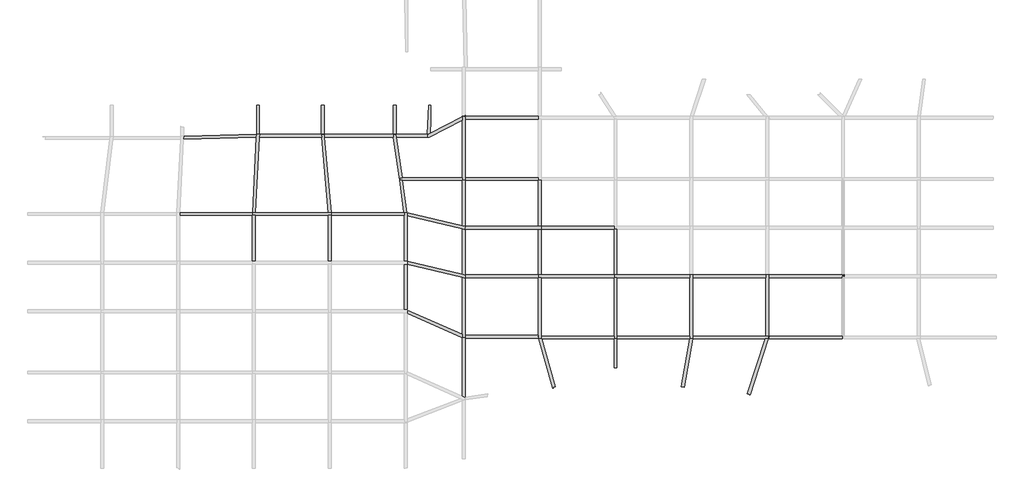
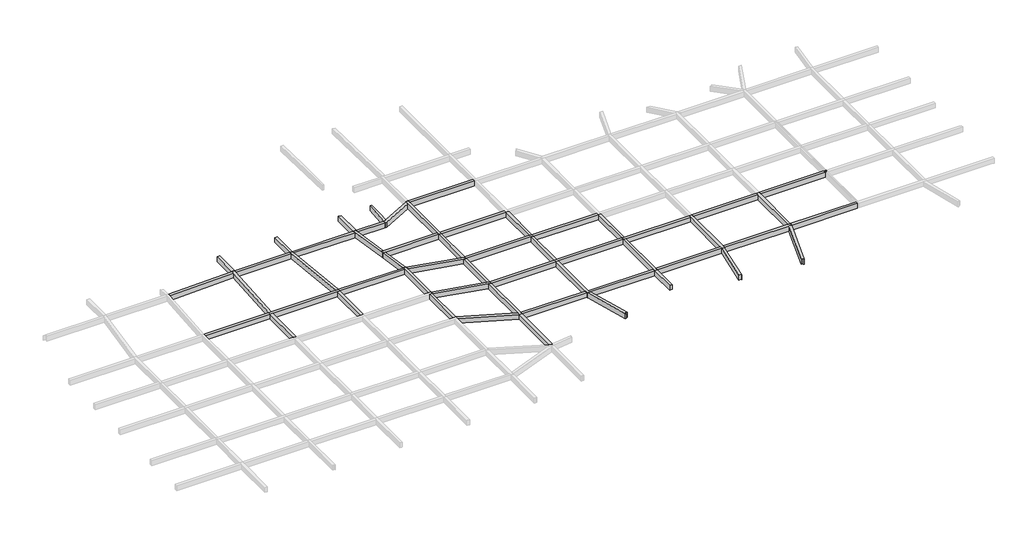
# One storey, part 8 of 15: 54 beams.
"""IFC4 building model written with IfcOpenShell, lengths in millimetres."""

from ifc_helpers import new_model, si_unit, frame, origin, place, context, project, spatial, polyline, outline, extrude, faceted_brep, element, save

model = new_model("IFC4")

# Units and contexts
model_context = context("Model", 3, world=origin())
ifc_project = project(units=[si_unit("LENGTHUNIT", "METRE", prefix="MILLI")], contexts=[model_context])

# Site, building, storey
site = spatial("IfcSite", under=ifc_project)
building = spatial("IfcBuilding", under=site)
storey = spatial("IfcBuildingStorey", under=building, Name="层高", Elevation=3300.0)

# Beams
placement = place(None, origin())
element("IfcBeam", 1, ObjectType="混凝土 - 矩形梁 : KL_beam", at=placement, inside=storey, context=model_context, shape_type="Brep", body=[
    faceted_brep([(131950.3009381, 116892.3894162, 3300.0), (131950.3009381, 116592.3894162, 3300.0), (132250.3009381, 116592.3894162, 3300.0), (139750.3009381, 116592.3894162, 3300.0), (140050.3009381, 116592.3894162, 3300.0), (140050.3009381, 116892.3894162, 3300.0), (140037.7506142, 116892.3894162, 3300.0), (139736.604663, 116892.3894162, 3300.0), (132258.3679569, 116892.3894162, 3300.0), (131957.9562531, 116892.3894162, 3300.0), (131950.3009381, 116592.3894162, 2700.0), (132250.3009381, 116592.3894162, 2700.0), (139750.3009381, 116592.3894162, 2700.0), (140050.3009381, 116592.3894162, 2700.0), (131950.3009381, 116892.3894162, 2700.0), (131957.9562531, 116892.3894162, 2700.0), (132258.3679569, 116892.3894162, 2700.0), (139736.604663, 116892.3894162, 2700.0), (140037.7506142, 116892.3894162, 2700.0), (140050.3009381, 116892.3894162, 2700.0)], [[[0, 1, 2, 3, 4, 5, 6, 7, 8, 9]], [[1, 10, 11, 12, 13, 4, 3, 2]], [[10, 14, 15, 16, 17, 18, 19, 13, 12, 11]], [[14, 0, 9, 8, 7, 6, 5, 19, 18, 17, 16, 15]], [[1, 0, 14, 10]], [[5, 4, 13, 19]]]),
])
element("IfcBeam", 2, ObjectType="混凝土 - 矩形梁 : KL_beam", at=placement, inside=storey, context=model_context, shape_type="SweptSolid", body=[
    extrude(outline(polyline([(131950.3009381, 116592.3894162), (132250.3009381, 116592.3894162), (132250.3009381, 111892.3894162), (131950.3009381, 111892.3894162), (131950.3009381, 116592.3894162)])), frame((0.0, 0.0, 2700.0), z_axis=(0.0, 0.0, 1.0), x_axis=(1.0, 0.0, 0.0)), (0.0, 0.0, 1.0), 600.0),
])
element("IfcBeam", 3, ObjectType="混凝土 - 矩形梁 : KL_beam", at=placement, inside=storey, context=model_context, shape_type="SweptSolid", body=[
    extrude(outline(polyline([(139750.3009381, 116592.3894162), (140050.3009381, 116592.3894162), (140050.3009381, 111892.3894162), (139750.3009381, 111892.3894162), (139750.3009381, 116592.3894162)])), frame((0.0, 0.0, 2700.0), z_axis=(0.0, 0.0, 1.0), x_axis=(1.0, 0.0, 0.0)), (0.0, 0.0, 1.0), 600.0),
])
element("IfcBeam", 4, ObjectType="混凝土 - 矩形梁 : KL_beam", at=placement, inside=storey, context=model_context, shape_type="Brep", body=[
    faceted_brep([(147850.2032763, 111592.3894162, 3300.0), (147550.2032763, 111592.3894162, 3300.0), (147550.2032763, 106892.3894162, 3300.0), (147850.2032763, 106892.3894162, 3300.0), (147850.2032763, 111553.3533934, 3300.0), (147550.2032763, 111592.3894162, 2700.0), (147550.2032763, 106892.3894162, 2700.0), (147850.2032763, 111592.3894162, 2700.0), (147850.2032763, 111553.3533934, 2700.0), (147850.2032763, 106892.3894162, 2700.0)], [[[0, 1, 2, 3, 4]], [[1, 5, 6, 2]], [[5, 7, 8, 9, 6]], [[7, 0, 4, 3, 9, 8]], [[1, 0, 7, 5]], [[3, 2, 6, 9]]]),
])
element("IfcBeam", 5, ObjectType="混凝土 - 矩形梁 : KL_beam", at=placement, inside=storey, context=model_context, shape_type="Brep", body=[
    faceted_brep([(147550.2032763, 111892.3894162, 2700.0), (147550.2032763, 111892.3894162, 3300.0), (147550.2032763, 116592.3894162, 3300.0), (147550.2032763, 116892.3894162, 3300.0), (147550.2032763, 116892.3894162, 2700.0), (147550.2032763, 116592.3894162, 2700.0), (147850.2032763, 111892.3894162, 3300.0), (147850.2032763, 111892.3894162, 2700.0), (147717.4740175, 116892.3894162, 3300.0), (147831.2059389, 116892.3894162, 3300.0), (147850.2032763, 116892.3894162, 3300.0), (147850.2032763, 116892.3894162, 2700.0), (147831.2059389, 116892.3894162, 2700.0), (147717.4740175, 116892.3894162, 2700.0), (147850.2032763, 116553.3533934, 3300.0), (147850.2032763, 116861.4143495, 3300.0), (147850.2032763, 116861.4143495, 2700.0), (147850.2032763, 116553.3533934, 2700.0)], [[[0, 1, 2, 3, 4, 5]], [[6, 1, 0, 7]], [[3, 8, 9, 10, 11, 12, 13, 4]], [[1, 6, 14, 15, 10, 9, 8, 3, 2]], [[7, 0, 5, 4, 13, 12, 11, 16, 17]], [[6, 7, 17, 16, 11, 10, 15, 14]]]),
])
element("IfcBeam", 6, ObjectType="混凝土 - 矩形梁 : KL_beam", at=placement, inside=storey, context=model_context, shape_type="Brep", body=[
    faceted_brep([(140050.3009381, 116892.3894162, 3300.0), (140050.3009381, 116592.3894162, 3300.0), (147550.2032763, 116592.3894162, 3300.0), (147550.2032763, 116892.3894162, 3300.0), (147528.451042, 116892.3894162, 3300.0), (140050.3009381, 116592.3894162, 2700.0), (147550.2032763, 116592.3894162, 2700.0), (140050.3009381, 116892.3894162, 2700.0), (147528.451042, 116892.3894162, 2700.0), (147550.2032763, 116892.3894162, 2700.0)], [[[0, 1, 2, 3, 4]], [[1, 5, 6, 2]], [[5, 7, 8, 9, 6]], [[7, 0, 4, 3, 9, 8]], [[1, 0, 7, 5]], [[3, 2, 6, 9]]]),
])
element("IfcBeam", 7, ObjectType="混凝土 - 矩形梁 : KL_beam", at=placement, inside=storey, context=model_context, shape_type="Brep", body=[
    faceted_brep([(147528.451042, 116892.3894162, 3300.0), (147550.2032763, 116892.3894162, 3300.0), (147717.4740175, 116892.3894162, 3300.0), (147522.2630229, 116937.9458643, 3300.0), (147717.4740175, 116892.3894162, 2700.0), (147522.2630229, 116937.9458643, 2700.0), (147550.2032763, 116892.3894162, 2700.0), (147528.451042, 116892.3894162, 2700.0)], [[[0, 1, 2, 3]], [[2, 4, 5, 3]], [[4, 6, 7, 5]], [[0, 7, 6, 4, 2, 1]], [[3, 5, 7, 0]]]),
    faceted_brep([(153782.1218117, 115169.0197936, 3300.0), (153683.0301969, 115192.1448334, 3300.0), (153550.3009381, 115223.1199001, 3300.0), (147850.2032763, 116553.3533934, 3300.0), (147850.2032763, 116553.3533934, 2700.0), (153550.3009381, 115223.1199001, 2700.0), (153683.0301969, 115192.1448334, 2700.0), (153782.1218117, 115169.0197936, 2700.0), (147850.2032763, 116861.4143495, 3300.0), (147850.2032763, 116861.4143495, 2700.0), (147850.2032763, 116592.3894162, 2700.0), (147850.2032763, 116592.3894162, 3300.0), (153787.5185091, 115192.1448334, 3300.0), (153850.3009381, 115461.1697666, 3300.0), (153550.3009381, 115531.1808562, 3300.0), (153850.3009381, 115461.1697666, 2700.0), (153550.3009381, 115531.1808562, 2700.0), (153787.5185091, 115192.1448334, 2700.0)], [[[0, 1, 2, 3, 4, 5, 6, 7]], [[8, 9, 10, 4, 3, 11]], [[3, 2, 1, 0, 12, 13, 14, 8, 11]], [[8, 14, 13, 15, 16, 9]], [[9, 16, 15, 17, 7, 6, 5, 4, 10]], [[0, 7, 17, 15, 13, 12]]]),
])
element("IfcBeam", 8, ObjectType="混凝土 - 矩形梁 : KL_beam", at=placement, inside=storey, context=model_context, shape_type="Brep", body=[
    faceted_brep([(147850.2032763, 111553.3533934, 3300.0), (147850.2032763, 111553.3533934, 2700.0), (153550.3009381, 110223.1199001, 2700.0), (153850.3009381, 110153.1088105, 2700.0), (153850.3009381, 110153.1088105, 3300.0), (153550.3009381, 110223.1199001, 3300.0), (147850.2032763, 111861.4143495, 3300.0), (147850.2032763, 111861.4143495, 2700.0), (147850.2032763, 111592.3894162, 2700.0), (147850.2032763, 111592.3894162, 3300.0), (153850.3009381, 110192.1448334, 3300.0), (153850.3009381, 110461.1697666, 3300.0), (153550.3009381, 110531.1808562, 3300.0), (153850.3009381, 110461.1697666, 2700.0), (153550.3009381, 110531.1808562, 2700.0), (153850.3009381, 110192.1448334, 2700.0)], [[[0, 1, 2, 3, 4, 5]], [[6, 7, 8, 1, 0, 9]], [[6, 9, 0, 5, 4, 10, 11, 12]], [[7, 6, 12, 11, 13, 14]], [[1, 8, 7, 14, 13, 15, 3, 2]], [[11, 10, 4, 3, 15, 13]]]),
])
element("IfcBeam", 9, ObjectType="混凝土 - 矩形梁 : KL_beam", at=placement, inside=storey, context=model_context, shape_type="Brep", body=[
    faceted_brep([(153550.3009381, 104021.0945528, 3300.0), (153850.3009381, 104021.0945528, 3300.0), (153850.3009381, 104269.2250309, 3300.0), (153850.3009381, 110153.1088105, 3300.0), (153550.3009381, 110223.1199001, 3300.0), (153550.3009381, 104348.5115934, 3300.0), (153850.3009381, 104021.0945528, 2700.0), (153850.3009381, 104269.2250309, 2700.0), (153850.3009381, 110153.1088105, 2700.0), (153550.3009381, 104021.0945528, 2700.0), (153550.3009381, 104348.5115934, 2700.0), (153550.3009381, 110223.1199001, 2700.0)], [[[0, 1, 2, 3, 4, 5]], [[1, 6, 7, 8, 3, 2]], [[6, 9, 10, 11, 8, 7]], [[9, 0, 5, 4, 11, 10]], [[4, 3, 8, 11]], [[0, 9, 6, 1]]]),
])
element("IfcBeam", 10, ObjectType="混凝土 - 矩形梁 : KL_beam", at=placement, inside=storey, context=model_context, shape_type="Brep", body=[
    faceted_brep([(147668.8470787, 106592.3894162, 3300.0), (147850.2032763, 106513.1028536, 3300.0), (153550.3009381, 104021.0945528, 3300.0), (153550.3009381, 104348.5115934, 3300.0), (147850.2032763, 106840.5198943, 3300.0), (147850.2032763, 106592.3894162, 3300.0), (147668.8470787, 106592.3894162, 2700.0), (147850.2032763, 106513.1028536, 2700.0), (153550.3009381, 104021.0945528, 2700.0), (147850.2032763, 106592.3894162, 2700.0), (147850.2032763, 106840.5198943, 2700.0), (153550.3009381, 104348.5115934, 2700.0)], [[[0, 1, 2, 3, 4, 5]], [[2, 1, 0, 6, 7, 8]], [[8, 7, 6, 9, 10, 11]], [[10, 4, 3, 11]], [[5, 9, 6, 0]], [[9, 5, 4, 10]], [[3, 2, 8, 11]]]),
])
element("IfcBeam", 11, ObjectType="混凝土 - 矩形梁 : KL_beam", at=placement, inside=storey, context=model_context, shape_type="Brep", body=[
    faceted_brep([(153850.3009381, 97839.1284443, 3300.0), (153850.3009381, 97914.6988398, 3300.0), (153850.3009381, 103969.2250309, 3300.0), (153850.3009381, 104021.0945528, 3300.0), (153550.3009381, 104021.0945528, 3300.0), (153550.3009381, 97974.1385386, 3300.0), (153550.3009381, 104021.0945528, 2700.0), (153550.3009381, 97974.1385386, 2700.0), (153850.3009381, 104021.0945528, 2700.0), (153850.3009381, 103969.2250309, 2700.0), (153850.3009381, 97914.6988398, 2700.0), (153850.3009381, 97839.1284443, 2700.0)], [[[0, 1, 2, 3, 4, 5]], [[4, 6, 7, 5]], [[8, 9, 10, 11, 7, 6]], [[3, 2, 1, 0, 11, 10, 9, 8]], [[4, 3, 8, 6]], [[0, 5, 7, 11]]]),
])
element("IfcBeam", 12, ObjectType="混凝土 - 矩形梁 : KL_beam", at=placement, inside=storey, context=model_context, shape_type="Brep", body=[
    faceted_brep([(177250.3009381, 110492.1448334, 3300.0), (176950.3009381, 110492.1448334, 3300.0), (176950.3009381, 110192.1448334, 3300.0), (176950.3009381, 104192.1448334, 3300.0), (176950.3009381, 103892.1448334, 3300.0), (177226.1658828, 103892.1448334, 3300.0), (177250.3009381, 103892.1448334, 3300.0), (177250.3009381, 104192.1448334, 3300.0), (177250.3009381, 110192.1448334, 3300.0), (177250.3009381, 110492.1448334, 2700.0), (177250.3009381, 103892.1448334, 2700.0), (177250.3009381, 104192.1448334, 2700.0), (177250.3009381, 110192.1448334, 2700.0), (176950.3009381, 110492.1448334, 2700.0), (177226.1658828, 103892.1448334, 2700.0), (176950.3009381, 103892.1448334, 2700.0), (176950.3009381, 104192.1448334, 2700.0), (176950.3009381, 110192.1448334, 2700.0)], [[[0, 1, 2, 3, 4, 5, 6, 7, 8]], [[9, 0, 8, 7, 6, 10, 11, 12]], [[13, 9, 12, 11, 10, 14, 15, 16, 17]], [[1, 13, 17, 16, 15, 4, 3, 2]], [[1, 0, 9, 13]], [[6, 5, 4, 15, 14, 10]]]),
])
element("IfcBeam", 13, ObjectType="混凝土 - 矩形梁 : KL_beam", at=placement, inside=storey, context=model_context, shape_type="Brep", body=[
    faceted_brep([(169150.3009381, 110492.1448334, 3300.0), (169150.3009381, 110192.1448334, 3300.0), (169450.3009381, 110192.1448334, 3300.0), (176950.3009381, 110192.1448334, 3300.0), (176950.3009381, 110492.1448334, 3300.0), (169450.3009381, 110492.1448334, 3300.0), (169150.3009381, 110492.1448334, 2700.0), (176950.3009381, 110492.1448334, 2700.0), (169450.3009381, 110492.1448334, 2700.0), (169150.3009381, 110192.1448334, 2700.0), (176950.3009381, 110192.1448334, 2700.0), (169450.3009381, 110192.1448334, 2700.0)], [[[0, 1, 2, 3, 4, 5]], [[6, 0, 5, 4, 7, 8]], [[9, 6, 8, 7, 10, 11]], [[1, 9, 11, 10, 3, 2]], [[4, 3, 10, 7]], [[1, 0, 6, 9]]]),
])
element("IfcBeam", 14, ObjectType="混凝土 - 矩形梁 : KL_beam", at=placement, inside=storey, context=model_context, shape_type="Brep", body=[
    faceted_brep([(169150.3009381, 103892.1448334, 3300.0), (169450.3009381, 103892.1448334, 3300.0), (169450.3009381, 104192.1448334, 3300.0), (169450.3009381, 110192.1448334, 3300.0), (169150.3009381, 110192.1448334, 3300.0), (169150.3009381, 104192.1448334, 3300.0), (169150.3009381, 103892.1448334, 2700.0), (169150.3009381, 110192.1448334, 2700.0), (169150.3009381, 104192.1448334, 2700.0), (169450.3009381, 103892.1448334, 2700.0), (169450.3009381, 110192.1448334, 2700.0), (169450.3009381, 104192.1448334, 2700.0)], [[[0, 1, 2, 3, 4, 5]], [[6, 0, 5, 4, 7, 8]], [[9, 6, 8, 7, 10, 11]], [[1, 9, 11, 10, 3, 2]], [[4, 3, 10, 7]], [[1, 0, 6, 9]]]),
])
element("IfcBeam", 15, ObjectType="混凝土 - 矩形梁 : KL_beam", at=placement, inside=storey, context=model_context, shape_type="Brep", body=[
    faceted_brep([(176950.3009381, 103892.1448334, 3300.0), (176950.3009381, 104192.1448334, 3300.0), (169450.3009381, 104192.1448334, 3300.0), (169450.3009381, 103892.1448334, 3300.0), (176921.5378992, 103892.1448334, 3300.0), (176950.3009381, 103892.1448334, 2700.0), (169450.3009381, 103892.1448334, 2700.0), (176921.5378992, 103892.1448334, 2700.0), (176950.3009381, 104192.1448334, 2700.0), (169450.3009381, 104192.1448334, 2700.0)], [[[0, 1, 2, 3, 4]], [[5, 0, 4, 3, 6, 7]], [[8, 5, 7, 6, 9]], [[1, 8, 9, 2]], [[1, 0, 5, 8]], [[3, 2, 9, 6]]]),
])
element("IfcBeam", 16, ObjectType="混凝土 - 矩形梁 : KL_beam", at=placement, inside=storey, context=model_context, shape_type="Brep", body=[
    faceted_brep([(177250.3009381, 104192.1448334, 3300.0), (177250.3009381, 103892.1448334, 3300.0), (184693.8920707, 103892.1448334, 3300.0), (185009.3078828, 103892.1448334, 3300.0), (185050.3009381, 103892.1448334, 3300.0), (185050.3009381, 104018.4043182, 3300.0), (185050.3009381, 104192.1448334, 3300.0), (184750.3009381, 104192.1448334, 3300.0), (177250.3009381, 103892.1448334, 2700.0), (184693.8920707, 103892.1448334, 2700.0), (185009.3078828, 103892.1448334, 2700.0), (185050.3009381, 103892.1448334, 2700.0), (177250.3009381, 104192.1448334, 2700.0), (184750.3009381, 104192.1448334, 2700.0), (185050.3009381, 104192.1448334, 2700.0), (185050.3009381, 104018.4043182, 2700.0)], [[[0, 1, 2, 3, 4, 5, 6, 7]], [[1, 8, 9, 10, 11, 4, 3, 2]], [[8, 12, 13, 14, 15, 11, 10, 9]], [[12, 0, 7, 6, 14, 13]], [[1, 0, 12, 8]], [[6, 5, 4, 11, 15, 14]]]),
])
element("IfcBeam", 17, ObjectType="混凝土 - 矩形梁 : KL_beam", at=placement, inside=storey, context=model_context, shape_type="Brep", body=[
    faceted_brep([(185050.3009381, 110492.1448334, 3300.0), (184750.3009381, 110492.1448334, 3300.0), (184750.3009381, 110192.1448334, 3300.0), (184750.3009381, 104192.1448334, 3300.0), (185050.3009381, 104192.1448334, 3300.0), (185050.3009381, 110192.1448334, 3300.0), (184750.3009381, 110492.1448334, 2700.0), (184750.3009381, 110192.1448334, 2700.0), (184750.3009381, 104192.1448334, 2700.0), (185050.3009381, 110492.1448334, 2700.0), (185050.3009381, 110192.1448334, 2700.0), (185050.3009381, 104192.1448334, 2700.0)], [[[0, 1, 2, 3, 4, 5]], [[1, 6, 7, 8, 3, 2]], [[6, 9, 10, 11, 8, 7]], [[9, 0, 5, 4, 11, 10]], [[4, 3, 8, 11]], [[1, 0, 9, 6]]]),
])
element("IfcBeam", 18, ObjectType="混凝土 - 矩形梁 : KL_beam", at=placement, inside=storey, context=model_context, shape_type="SweptSolid", body=[
    extrude(outline(polyline([(177250.3009381, 110192.1448334), (177250.3009381, 110492.1448334), (184750.3009381, 110492.1448334), (184750.3009381, 110192.1448334), (177250.3009381, 110192.1448334)])), frame((0.0, 0.0, 2700.0), z_axis=(0.0, 0.0, 1.0), x_axis=(1.0, 0.0, 0.0)), (0.0, 0.0, 1.0), 600.0),
])
element("IfcBeam", 19, ObjectType="混凝土 - 矩形梁 : KL_beam", at=placement, inside=storey, context=model_context, shape_type="SweptSolid", body=[
    extrude(outline(polyline([(169450.3009381, 110492.1448334), (169150.3009381, 110492.1448334), (169150.3009381, 115192.1448334), (169450.3009381, 115192.1448334), (169450.3009381, 110492.1448334)])), frame((0.0, 0.0, 2700.0), z_axis=(0.0, 0.0, 1.0), x_axis=(1.0, 0.0, 0.0)), (0.0, 0.0, 1.0), 600.0),
])
element("IfcBeam", 20, ObjectType="混凝土 - 矩形梁 : KL_beam", at=placement, inside=storey, context=model_context, shape_type="Brep", body=[
    faceted_brep([(161350.3009383, 110492.1448334, 3300.0), (161350.3009383, 110192.1448334, 3300.0), (161650.3009383, 110192.1448334, 3300.0), (169150.3009381, 110192.1448334, 3300.0), (169150.3009381, 110492.1448334, 3300.0), (161650.3009383, 110492.1448334, 3300.0), (161350.3009383, 110192.1448334, 2700.0), (161650.3009383, 110192.1448334, 2700.0), (169150.3009381, 110192.1448334, 2700.0), (161350.3009383, 110492.1448334, 2700.0), (161650.3009383, 110492.1448334, 2700.0), (169150.3009381, 110492.1448334, 2700.0)], [[[0, 1, 2, 3, 4, 5]], [[1, 6, 7, 8, 3, 2]], [[6, 9, 10, 11, 8, 7]], [[9, 0, 5, 4, 11, 10]], [[4, 3, 8, 11]], [[1, 0, 9, 6]]]),
])
element("IfcBeam", 21, ObjectType="混凝土 - 矩形梁 : KL_beam", at=placement, inside=storey, context=model_context, shape_type="Brep", body=[
    faceted_brep([(161350.3009383, 103892.1448334, 3300.0), (161387.2678308, 103892.1448334, 3300.0), (161650.3009383, 103892.1448334, 3300.0), (161650.3009383, 104192.1448334, 3300.0), (161650.3009383, 110192.1448334, 3300.0), (161350.3009383, 110192.1448334, 3300.0), (161350.3009383, 104269.2250309, 3300.0), (161350.3009383, 104208.7009636, 3300.0), (161350.3009383, 104021.0637081, 3300.0), (161350.3009383, 103969.2250309, 3300.0), (161650.3009383, 103892.1448334, 2700.0), (161650.3009383, 104192.1448334, 2700.0), (161650.3009383, 110192.1448334, 2700.0), (161387.2678308, 103892.1448334, 2700.0), (161350.3009383, 103892.1448334, 2700.0), (161350.3009383, 103969.2250309, 2700.0), (161350.3009383, 104021.0637081, 2700.0), (161350.3009383, 104208.7009636, 2700.0), (161350.3009383, 104269.2250309, 2700.0), (161350.3009383, 110192.1448334, 2700.0)], [[[0, 1, 2, 3, 4, 5, 6, 7, 8, 9]], [[2, 10, 11, 12, 4, 3]], [[10, 13, 14, 15, 16, 17, 18, 19, 12, 11]], [[14, 0, 9, 8, 7, 6, 5, 19, 18, 17, 16, 15]], [[5, 4, 12, 19]], [[2, 1, 0, 14, 13, 10]]]),
])
element("IfcBeam", 22, ObjectType="混凝土 - 矩形梁 : KL_beam", at=placement, inside=storey, context=model_context, shape_type="Brep", body=[
    faceted_brep([(169150.3009381, 103892.1448334, 3300.0), (169150.3009381, 104192.1448334, 3300.0), (161650.3009383, 104192.1448334, 3300.0), (161650.3009383, 103892.1448334, 3300.0), (161699.3576615, 103892.1448334, 3300.0), (169150.3009381, 104192.1448334, 2700.0), (161650.3009383, 104192.1448334, 2700.0), (169150.3009381, 103892.1448334, 2700.0), (161699.3576615, 103892.1448334, 2700.0), (161650.3009383, 103892.1448334, 2700.0)], [[[0, 1, 2, 3, 4]], [[1, 5, 6, 2]], [[5, 7, 8, 9, 6]], [[7, 0, 4, 3, 9, 8]], [[1, 0, 7, 5]], [[3, 2, 6, 9]]]),
])
element("IfcBeam", 23, ObjectType="混凝土 - 矩形梁 : KL_beam", at=placement, inside=storey, context=model_context, shape_type="Brep", body=[
    faceted_brep([(161699.3576615, 103892.1448334, 3300.0), (161650.3009383, 103892.1448334, 3300.0), (161387.2678308, 103892.1448334, 3300.0), (162838.6902887, 98830.4331897, 3300.0), (162917.5304809, 98830.4331897, 3300.0), (162917.5304809, 98950.4331897, 3300.0), (163116.3706731, 98950.4331897, 3300.0), (161387.2678308, 103892.1448334, 2700.0), (162838.6902887, 98830.4331897, 2700.0), (161650.3009383, 103892.1448334, 2700.0), (161699.3576615, 103892.1448334, 2700.0), (163116.3706731, 98950.4331897, 2700.0), (162917.5304809, 98950.4331897, 2700.0), (162917.5304809, 98830.4331897, 2700.0)], [[[0, 1, 2, 3, 4, 5, 6]], [[2, 7, 8, 3]], [[7, 9, 10, 11, 12, 13, 8]], [[10, 0, 6, 11]], [[7, 2, 1, 0, 10, 9]], [[3, 8, 13, 4]], [[5, 12, 11, 6]], [[12, 5, 4, 13]]]),
    faceted_brep([(161300.5846401, 104194.4450445, 2700.0), (161300.5846401, 104194.4450445, 3300.0), (161350.3009383, 104208.7009636, 3300.0), (161350.3009383, 104208.7009636, 2700.0), (161350.3009383, 104021.0637081, 3300.0), (161350.3009383, 104021.0637081, 2700.0), (161350.3009383, 104192.1448334, 2700.0), (161350.3009383, 104192.1448334, 3300.0)], [[[0, 1, 2, 3]], [[4, 5, 6, 3, 2, 7]], [[2, 1, 4, 7]], [[1, 0, 5, 4]], [[0, 3, 6, 5]]]),
])
element("IfcBeam", 24, ObjectType="混凝土 - 矩形梁 : KL_beam", at=placement, inside=storey, context=model_context, shape_type="SweptSolid", body=[
    extrude(outline(polyline([(169150.3009381, 103892.1448334), (169450.3009381, 103892.1448334), (169450.3009381, 100902.3018651), (169150.3009381, 100902.3018651), (169150.3009381, 103892.1448334)])), frame((0.0, 0.0, 2700.0), z_axis=(0.0, 0.0, 1.0), x_axis=(1.0, 0.0, 0.0)), (0.0, 0.0, 1.0), 600.0),
])
element("IfcBeam", 25, ObjectType="混凝土 - 矩形梁 : KL_beam", at=placement, inside=storey, context=model_context, shape_type="Brep", body=[
    faceted_brep([(177226.1658828, 103892.1448334, 3300.0), (176950.3009381, 103892.1448334, 3300.0), (176921.5378992, 103892.1448334, 3300.0), (176050.1808056, 98950.4331897, 3300.0), (176349.86269, 98950.4331897, 3300.0), (176349.86269, 98922.3824677, 3300.0), (176921.5378992, 103892.1448334, 2700.0), (176050.1808056, 98950.4331897, 2700.0), (176950.3009381, 103892.1448334, 2700.0), (177226.1658828, 103892.1448334, 2700.0), (176349.86269, 98922.3824677, 2700.0), (176349.86269, 98950.4331897, 2700.0)], [[[0, 1, 2, 3, 4, 5]], [[2, 6, 7, 3]], [[6, 8, 9, 10, 11, 7]], [[9, 0, 5, 10]], [[0, 9, 8, 6, 2, 1]], [[3, 7, 11, 4]], [[4, 11, 10, 5]]]),
])
element("IfcBeam", 26, ObjectType="混凝土 - 矩形梁 : KL_beam", at=placement, inside=storey, context=model_context, shape_type="Brep", body=[
    faceted_brep([(185050.3009381, 104192.1448334, 3300.0), (185050.3009381, 104018.4043182, 3300.0), (185106.7098056, 104192.1448334, 3300.0), (185050.3009381, 104018.4043182, 2700.0), (185106.7098056, 104192.1448334, 2700.0), (185050.3009381, 104192.1448334, 2700.0)], [[[0, 1, 2]], [[1, 3, 4, 2]], [[3, 5, 4]], [[5, 0, 2, 4]], [[1, 0, 5, 3]]]),
    faceted_brep([(184693.8920707, 103892.1448334, 3300.0), (184693.8920707, 103892.1448334, 2700.0), (182862.1801986, 98250.4331897, 2700.0), (182862.1801986, 98250.4331897, 3300.0), (185009.3078828, 103892.1448334, 3300.0), (185009.3078828, 103892.1448334, 2700.0), (184750.3009381, 103892.1448334, 2700.0), (184750.3009381, 103892.1448334, 3300.0), (183060.4077201, 98250.4331897, 3300.0), (183060.4077201, 98130.4331897, 3300.0), (183138.6352416, 98130.4331897, 3300.0), (183138.6352416, 98130.4331897, 2700.0), (183060.4077201, 98130.4331897, 2700.0), (183060.4077201, 98250.4331897, 2700.0)], [[[0, 1, 2, 3]], [[4, 5, 6, 1, 0, 7]], [[7, 0, 3, 8, 9, 10, 4]], [[5, 4, 10, 11]], [[6, 5, 11, 12, 13, 2, 1]], [[11, 10, 9, 12]], [[8, 13, 12, 9]], [[13, 8, 3, 2]]]),
])
element("IfcBeam", 27, ObjectType="混凝土 - 矩形梁 : KL_beam", at=placement, inside=storey, context=model_context, shape_type="Brep", body=[
    faceted_brep([(185050.3009381, 104018.4043182, 3300.0), (185050.3009381, 103892.1448334, 3300.0), (192640.3009401, 103892.1448334, 3300.0), (192640.3009401, 104192.1448334, 3300.0), (192550.3215993, 104192.1448334, 3300.0), (185106.7098056, 104192.1448334, 3300.0), (185050.3009381, 103892.1448334, 2700.0), (192640.3009401, 103892.1448334, 2700.0), (185050.3009381, 104018.4043182, 2700.0), (185106.7098056, 104192.1448334, 2700.0), (192550.3215993, 104192.1448334, 2700.0), (192640.3009401, 104192.1448334, 2700.0)], [[[0, 1, 2, 3, 4, 5]], [[1, 6, 7, 2]], [[6, 8, 9, 10, 11, 7]], [[9, 5, 4, 3, 11, 10]], [[6, 1, 0, 8]], [[0, 5, 9, 8]], [[3, 2, 7, 11]]]),
])
element("IfcBeam", 28, ObjectType="混凝土 - 矩形梁 : KL_beam", at=placement, inside=storey, context=model_context, shape_type="Brep", body=[
    faceted_brep([(192850.3009401, 110342.1448334, 3300.0), (192850.3009401, 110492.1448334, 3300.0), (192760.3009401, 110492.1448334, 3300.0), (192760.3009401, 110342.1448334, 3300.0), (192850.3009401, 110492.1448334, 2700.0), (192850.3009401, 110342.1448334, 2700.0), (192760.3009401, 110342.1448334, 2700.0), (192760.3009401, 110492.1448334, 2700.0)], [[[0, 1, 2, 3]], [[4, 5, 6, 7]], [[1, 4, 7, 2]], [[4, 1, 0, 5]], [[3, 2, 7, 6]], [[5, 0, 3, 6]]]),
    faceted_brep([(185050.3009381, 110192.1448334, 3300.0), (185050.3009381, 110192.1448334, 2700.0), (192550.3215993, 110192.1448334, 2700.0), (192550.3215993, 110192.1448334, 3300.0), (185050.3009381, 110492.1448334, 3300.0), (185050.3009381, 110492.1448334, 2700.0), (192550.3215993, 110342.1448334, 3300.0), (192550.3215993, 110342.1448334, 2700.0), (192640.3009401, 110342.1448334, 2700.0), (192640.3009401, 110342.1448334, 3300.0), (192640.3009401, 110492.1448334, 3300.0), (192640.3009401, 110492.1448334, 2700.0), (192550.3009401, 110492.1448334, 3300.0), (192550.3009401, 110492.1448334, 2700.0)], [[[0, 1, 2, 3]], [[0, 4, 5, 1]], [[6, 3, 2, 7]], [[6, 7, 8, 9]], [[10, 9, 8, 11]], [[4, 0, 3, 6, 9, 10, 12]], [[1, 5, 13, 11, 8, 7, 2]], [[5, 4, 12, 10, 11, 13]]]),
])
element("IfcBeam", 29, ObjectType="混凝土 - 矩形梁 : KL_beam", at=placement, inside=storey, context=model_context, shape_type="Brep", body=[
    faceted_brep([(153850.3009381, 126792.1448334, 3300.0), (153664.2891243, 126792.1448334, 3300.0), (153550.3009381, 126792.1448334, 3300.0), (153550.3009381, 126734.0649516, 3300.0), (153550.3009381, 126397.3670803, 3300.0), (153550.3009381, 120492.1448334, 3300.0), (153550.3009381, 120192.1448334, 3300.0), (153850.3009381, 120192.1448334, 3300.0), (153850.3009381, 120492.1448334, 3300.0), (153850.3009381, 126492.1448334, 3300.0), (153550.3009381, 126792.1448334, 2700.0), (153550.3009381, 126734.0649516, 2700.0), (153550.3009381, 126397.3670803, 2700.0), (153550.3009381, 120492.1448334, 2700.0), (153550.3009381, 120192.1448334, 2700.0), (153664.2891243, 126792.1448334, 2700.0), (153850.3009381, 126792.1448334, 2700.0), (153850.3009381, 126492.1448334, 2700.0), (153850.3009381, 120492.1448334, 2700.0), (153850.3009381, 120192.1448334, 2700.0)], [[[0, 1, 2, 3, 4, 5, 6, 7, 8, 9]], [[2, 10, 11, 12, 13, 14, 6, 5, 4, 3]], [[10, 15, 16, 17, 18, 19, 14, 13, 12, 11]], [[16, 0, 9, 8, 7, 19, 18, 17]], [[2, 1, 0, 16, 15, 10]], [[7, 6, 14, 19]]]),
])
element("IfcBeam", 30, ObjectType="混凝土 - 矩形梁 : KL_beam", at=placement, inside=storey, context=model_context, shape_type="SweptSolid", body=[
    extrude(outline(polyline([(161350.3009383, 126792.1448334), (161350.3009383, 126492.1448334), (153850.3009381, 126492.1448334), (153850.3009381, 126792.1448334), (161350.3009383, 126792.1448334)])), frame((0.0, 0.0, 2700.0), z_axis=(0.0, 0.0, 1.0), x_axis=(1.0, 0.0, 0.0)), (0.0, 0.0, 1.0), 600.0),
])
element("IfcBeam", 31, ObjectType="混凝土 - 矩形梁 : KL_beam", at=placement, inside=storey, context=model_context, shape_type="SweptSolid", body=[
    extrude(outline(polyline([(161350.3009383, 120492.1448334), (161350.3009383, 120192.1448334), (153850.3009381, 120192.1448334), (153850.3009381, 120492.1448334), (161350.3009383, 120492.1448334)])), frame((0.0, 0.0, 2700.0), z_axis=(0.0, 0.0, 1.0), x_axis=(1.0, 0.0, 0.0)), (0.0, 0.0, 1.0), 600.0),
])
element("IfcBeam", 32, ObjectType="混凝土 - 矩形梁 : KL_beam", at=placement, inside=storey, context=model_context, shape_type="Brep", body=[
    faceted_brep([(147080.2389772, 120492.1448334, 3300.0), (147080.2389772, 120196.4827327, 3300.0), (147080.2389772, 120192.1448334, 3300.0), (147382.9938741, 120192.1448334, 3300.0), (153550.3009381, 120192.1448334, 3300.0), (153550.3009381, 120492.1448334, 3300.0), (147341.6346506, 120492.1448334, 3300.0), (147080.2389772, 120192.1448334, 2700.0), (147382.9938741, 120192.1448334, 2700.0), (153550.3009381, 120192.1448334, 2700.0), (147080.2389772, 120196.4827327, 2700.0), (147080.2389772, 120492.1448334, 2700.0), (147341.6346506, 120492.1448334, 2700.0), (153550.3009381, 120492.1448334, 2700.0)], [[[0, 1, 2, 3, 4, 5, 6]], [[2, 7, 8, 9, 4, 3]], [[7, 10, 11, 12, 13, 9, 8]], [[11, 0, 6, 5, 13, 12]], [[5, 4, 9, 13]], [[0, 11, 10, 7, 2, 1]]]),
])
element("IfcBeam", 33, ObjectType="混凝土 - 矩形梁 : KL_beam", at=placement, inside=storey, context=model_context, shape_type="SweptSolid", body=[
    extrude(outline(polyline([(147831.2059389, 116892.3894162), (147717.4740175, 116892.3894162), (147522.2630229, 116937.9458643), (147080.2389772, 120192.1448334), (147382.9938741, 120192.1448334), (147831.2059389, 116892.3894162)])), frame((0.0, 0.0, 2700.0), z_axis=(0.0, 0.0, 1.0), x_axis=(1.0, 0.0, 0.0)), (0.0, 0.0, 1.0), 600.0),
])
element("IfcBeam", 34, ObjectType="混凝土 - 矩形梁 : KL_beam", at=placement, inside=storey, context=model_context, shape_type="Brep", body=[
    faceted_brep([(153550.3009381, 115531.1808562, 3300.0), (153850.3009381, 115461.1697666, 3300.0), (153850.3009381, 115492.1448334, 3300.0), (153850.3009381, 120192.1448334, 3300.0), (153550.3009381, 120192.1448334, 3300.0), (153850.3009381, 115461.1697666, 2700.0), (153850.3009381, 115492.1448334, 2700.0), (153850.3009381, 120192.1448334, 2700.0), (153550.3009381, 115531.1808562, 2700.0), (153550.3009381, 120192.1448334, 2700.0)], [[[0, 1, 2, 3, 4]], [[1, 5, 6, 7, 3, 2]], [[5, 8, 9, 7, 6]], [[8, 0, 4, 9]], [[1, 0, 8, 5]], [[4, 3, 7, 9]]]),
])
element("IfcBeam", 35, ObjectType="混凝土 - 矩形梁 : KL_beam", at=placement, inside=storey, context=model_context, shape_type="Brep", body=[
    faceted_brep([(153850.3009381, 115461.1697666, 3300.0), (153787.5185091, 115192.1448334, 3300.0), (153850.3009381, 115192.1448334, 3300.0), (161350.3009383, 115192.1448334, 3300.0), (161650.3009383, 115192.1448334, 3300.0), (161650.3009383, 115492.1448334, 3300.0), (161350.3009383, 115492.1448334, 3300.0), (153850.3009381, 115492.1448334, 3300.0), (161650.3009383, 115492.1448334, 2700.0), (161350.3009383, 115492.1448334, 2700.0), (153850.3009381, 115492.1448334, 2700.0), (153787.5185091, 115192.1448334, 2700.0), (153850.3009381, 115461.1697666, 2700.0), (161650.3009383, 115192.1448334, 2700.0), (161350.3009383, 115192.1448334, 2700.0), (153850.3009381, 115192.1448334, 2700.0)], [[[0, 1, 2, 3, 4, 5, 6, 7]], [[5, 8, 9, 10, 7, 6]], [[11, 12, 10, 9, 8, 13, 14, 15]], [[1, 11, 15, 14, 13, 4, 3, 2]], [[1, 0, 12, 11]], [[0, 7, 10, 12]], [[5, 4, 13, 8]]]),
    faceted_brep([(153550.3009381, 115223.1199001, 3300.0), (153683.0301969, 115192.1448334, 3300.0), (153683.0301969, 115192.1448334, 2700.0), (153550.3009381, 115223.1199001, 2700.0), (153550.3009381, 115192.1448334, 2700.0), (153550.3009381, 115192.1448334, 3300.0)], [[[0, 1, 2, 3]], [[4, 5, 0, 3]], [[1, 0, 5]], [[3, 2, 4]], [[2, 1, 5, 4]]]),
])
element("IfcBeam", 36, ObjectType="混凝土 - 矩形梁 : KL_beam", at=placement, inside=storey, context=model_context, shape_type="Brep", body=[
    faceted_brep([(153787.5185091, 115192.1448334, 3300.0), (153782.1218117, 115169.0197936, 3300.0), (153683.0301969, 115192.1448334, 3300.0), (153550.3009381, 115192.1448334, 3300.0), (153550.3009381, 110531.1808562, 3300.0), (153850.3009381, 110461.1697666, 3300.0), (153850.3009381, 110492.1448334, 3300.0), (153850.3009381, 115192.1448334, 3300.0), (153550.3009381, 115192.1448334, 2700.0), (153550.3009381, 110531.1808562, 2700.0), (153683.0301969, 115192.1448334, 2700.0), (153782.1218117, 115169.0197936, 2700.0), (153787.5185091, 115192.1448334, 2700.0), (153850.3009381, 115192.1448334, 2700.0), (153850.3009381, 110492.1448334, 2700.0), (153850.3009381, 110461.1697666, 2700.0)], [[[0, 1, 2, 3, 4, 5, 6, 7]], [[3, 8, 9, 4]], [[10, 11, 12, 13, 14, 15, 9, 8]], [[13, 7, 6, 5, 15, 14]], [[1, 11, 10, 2]], [[11, 1, 0, 12]], [[3, 2, 10, 8]], [[0, 7, 13, 12]], [[5, 4, 9, 15]]]),
])
element("IfcBeam", 37, ObjectType="混凝土 - 矩形梁 : KL_beam", at=placement, inside=storey, context=model_context, shape_type="Brep", body=[
    faceted_brep([(153850.3009381, 110492.1448334, 2700.0), (153850.3009381, 110492.1448334, 3300.0), (161350.3009383, 110492.1448334, 3300.0), (161350.3009383, 110492.1448334, 2700.0), (153850.3009381, 110192.1448334, 2700.0), (153850.3009381, 110192.1448334, 3300.0), (153850.3009381, 110461.1697666, 3300.0), (153850.3009381, 110461.1697666, 2700.0), (161350.3009383, 110192.1448334, 3300.0), (161350.3009383, 110192.1448334, 2700.0)], [[[0, 1, 2, 3]], [[4, 5, 6, 1, 0, 7]], [[1, 6, 5, 8, 2]], [[5, 4, 9, 8]], [[4, 7, 0, 3, 9]], [[3, 2, 8, 9]]]),
])
element("IfcBeam", 38, ObjectType="混凝土 - 矩形梁 : KL_beam", at=placement, inside=storey, context=model_context, shape_type="SweptSolid", body=[
    extrude(outline(polyline([(161650.3009383, 110492.1448334), (161350.3009383, 110492.1448334), (161350.3009383, 115192.1448334), (161650.3009383, 115192.1448334), (161650.3009383, 110492.1448334)])), frame((0.0, 0.0, 2700.0), z_axis=(0.0, 0.0, 1.0), x_axis=(1.0, 0.0, 0.0)), (0.0, 0.0, 1.0), 600.0),
])
element("IfcBeam", 39, ObjectType="混凝土 - 矩形梁 : KL_beam", at=placement, inside=storey, context=model_context, shape_type="Brep", body=[
    faceted_brep([(153850.3009381, 104269.2250309, 2700.0), (153850.3009381, 104269.2250309, 3300.0), (161350.3009383, 104269.2250309, 3300.0), (161350.3009383, 104269.2250309, 2700.0), (153850.3009381, 104021.0945528, 2700.0), (153850.3009381, 103969.2250309, 2700.0), (153850.3009381, 103969.2250309, 3300.0), (153850.3009381, 104021.0945528, 3300.0), (161350.3009383, 104208.7009636, 3300.0), (161350.3009383, 104208.7009636, 2700.0), (161350.3009383, 103969.2250309, 3300.0), (161350.3009383, 104021.0637081, 3300.0), (161300.5846401, 104194.4450445, 3300.0), (161350.3009383, 103969.2250309, 2700.0), (161300.5846401, 104194.4450445, 2700.0), (161350.3009383, 104021.0637081, 2700.0)], [[[0, 1, 2, 3]], [[1, 0, 4, 5, 6, 7]], [[3, 2, 8, 9]], [[1, 7, 6, 10, 11, 12, 8, 2]], [[6, 5, 13, 10]], [[5, 4, 0, 3, 9, 14, 15, 13]], [[14, 12, 11, 15]], [[12, 14, 9, 8]], [[10, 13, 15, 11]]]),
])
element("IfcBeam", 40, ObjectType="混凝土 - 矩形梁 : KL_beam", at=placement, inside=storey, context=model_context, shape_type="SweptSolid", body=[
    extrude(outline(polyline([(124450.3009381, 116592.3894162), (124450.3009381, 116738.461528), (124458.3679569, 116892.3894162), (131950.3009381, 116892.3894162), (131950.3009381, 116592.3894162), (124450.3009381, 116592.3894162)])), frame((0.0, 0.0, 2700.0), z_axis=(0.0, 0.0, 1.0), x_axis=(1.0, 0.0, 0.0)), (0.0, 0.0, 1.0), 600.0),
])
element("IfcBeam", 41, ObjectType="混凝土 - 矩形梁 : KL_beam", at=placement, inside=storey, context=model_context, shape_type="Brep", body=[
    faceted_brep([(131957.9562531, 116892.3894162, 3300.0), (132250.3009381, 116892.3894162, 3300.0), (132258.3679569, 116892.3894162, 3300.0), (132664.8406872, 124648.3511427, 3300.0), (132680.563021, 124948.3511427, 3300.0), (132672.4960022, 124948.3511427, 3300.0), (132520.2611111, 124948.3511427, 3300.0), (132380.1513172, 124948.3511427, 3300.0), (132379.9321201, 124944.1686142, 3300.0), (132364.1781965, 124643.5658433, 3300.0), (132258.3679569, 116892.3894162, 2700.0), (132664.8406872, 124648.3511427, 2700.0), (132680.563021, 124948.3511427, 2700.0), (132250.3009381, 116892.3894162, 2700.0), (131957.9562531, 116892.3894162, 2700.0), (132364.1781965, 124643.5658433, 2700.0), (132379.9321201, 124944.1686142, 2700.0), (132380.1513172, 124948.3511427, 2700.0), (132520.2611111, 124948.3511427, 2700.0), (132672.4960022, 124948.3511427, 2700.0)], [[[0, 1, 2, 3, 4, 5, 6, 7, 8, 9]], [[2, 10, 11, 12, 4, 3]], [[10, 13, 14, 15, 16, 17, 18, 19, 12, 11]], [[14, 0, 9, 8, 7, 17, 16, 15]], [[10, 2, 1, 0, 14, 13]], [[7, 6, 5, 4, 12, 19, 18, 17]]]),
])
element("IfcBeam", 42, ObjectType="混凝土 - 矩形梁 : KL_beam", at=placement, inside=storey, context=model_context, shape_type="Brep", body=[
    faceted_brep([(139034.0868799, 124922.2044199, 3300.0), (139058.0459371, 124648.3511427, 3300.0), (139736.604663, 116892.3894162, 3300.0), (139750.3009381, 116892.3894162, 3300.0), (140037.7506142, 116892.3894162, 3300.0), (139359.1918884, 124648.3511427, 3300.0), (139332.9452894, 124948.3511427, 3300.0), (140037.7506142, 116892.3894162, 2700.0), (139359.1918884, 124648.3511427, 2700.0), (139332.9452894, 124948.3511427, 2700.0), (139750.3009381, 116892.3894162, 2700.0), (139736.604663, 116892.3894162, 2700.0), (139058.0459371, 124648.3511427, 2700.0), (139034.0868799, 124922.2044199, 2700.0)], [[[0, 1, 2, 3, 4, 5, 6]], [[6, 5, 4, 7, 8, 9]], [[9, 8, 7, 10, 11, 12, 13]], [[2, 1, 0, 13, 12, 11]], [[7, 4, 3, 2, 11, 10]], [[0, 6, 9, 13]]]),
])
element("IfcBeam", 43, ObjectType="混凝土 - 矩形梁 : KL_beam", at=placement, inside=storey, context=model_context, shape_type="Brep", body=[
    faceted_brep([(146418.2752756, 124906.5992124, 3300.0), (146454.5696749, 124648.3511427, 3300.0), (147080.2389772, 120196.4827327, 3300.0), (147080.2389772, 120492.1448334, 3300.0), (147341.6346506, 120492.1448334, 3300.0), (146757.5179467, 124648.3511427, 3300.0), (146715.3556962, 124948.3511427, 3300.0), (147341.6346506, 120492.1448334, 2700.0), (146757.5179467, 124648.3511427, 2700.0), (146715.3556962, 124948.3511427, 2700.0), (147080.2389772, 120492.1448334, 2700.0), (147080.2389772, 120196.4827327, 2700.0), (146454.5696749, 124648.3511427, 2700.0), (146418.2752756, 124906.5992124, 2700.0)], [[[0, 1, 2, 3, 4, 5, 6]], [[6, 5, 4, 7, 8, 9]], [[9, 8, 7, 10, 11, 12, 13]], [[2, 1, 0, 13, 12, 11]], [[3, 10, 7, 4]], [[10, 3, 2, 11]], [[0, 6, 9, 13]]]),
])
element("IfcBeam", 44, ObjectType="混凝土 - 矩形梁 : KL_beam", at=placement, inside=storey, context=model_context, shape_type="Brep", body=[
    faceted_brep([(149923.5866775, 124648.3511427, 3300.0), (150117.6638847, 124648.3511427, 3300.0), (153550.3009381, 126397.3670803, 3300.0), (153550.3009381, 126492.1448334, 3300.0), (153550.3009381, 126734.0649516, 3300.0), (150245.0410364, 125049.9509145, 3300.0), (150045.640257, 124948.3511427, 3300.0), (149936.3891524, 124892.6849245, 3300.0), (153550.3009381, 126734.0649516, 2700.0), (150245.0410364, 125049.9509145, 2700.0), (150045.640257, 124948.3511427, 2700.0), (149936.3891524, 124892.6849245, 2700.0), (150117.6638847, 124648.3511427, 2700.0), (149923.5866775, 124648.3511427, 2700.0), (153550.3009381, 126492.1448334, 2700.0), (153550.3009381, 126397.3670803, 2700.0)], [[[0, 1, 2, 3, 4, 5, 6, 7]], [[4, 8, 9, 10, 11, 7, 6, 5]], [[12, 13, 11, 10, 9, 8, 14, 15]], [[15, 2, 1, 12]], [[8, 4, 3, 2, 15, 14]], [[1, 0, 13, 12]], [[13, 0, 7, 11]]]),
    faceted_brep([(153850.3009381, 126886.9225864, 2700.0), (153850.3009381, 126886.9225864, 3300.0), (153850.3009381, 126792.1448334, 3300.0), (153850.3009381, 126792.1448334, 2700.0), (153664.2891243, 126792.1448334, 3300.0), (153664.2891243, 126792.1448334, 2700.0)], [[[0, 1, 2, 3]], [[2, 4, 5, 3]], [[4, 2, 1]], [[1, 0, 5, 4]], [[3, 5, 0]]]),
])
element("IfcBeam", 45, ObjectType="混凝土 - 矩形梁 : KL_beam", at=placement, inside=storey, context=model_context, shape_type="Brep", body=[
    faceted_brep([(146715.3556962, 124948.3511427, 3300.0), (146757.5179467, 124648.3511427, 3300.0), (149923.5866775, 124648.3511427, 3300.0), (149936.3891524, 124892.6849245, 3300.0), (150045.640257, 124948.3511427, 3300.0), (149939.3059221, 124948.3511427, 3300.0), (146734.9626856, 124948.3511427, 3300.0), (146757.5179467, 124648.3511427, 2700.0), (149923.5866775, 124648.3511427, 2700.0), (146715.3556962, 124948.3511427, 2700.0), (146734.9626856, 124948.3511427, 2700.0), (149939.3059221, 124948.3511427, 2700.0), (150045.640257, 124948.3511427, 2700.0), (149936.3891524, 124892.6849245, 2700.0)], [[[0, 1, 2, 3, 4, 5, 6]], [[1, 7, 8, 2]], [[7, 9, 10, 11, 12, 13, 8]], [[9, 0, 6, 5, 4, 12, 11, 10]], [[1, 0, 9, 7]], [[3, 13, 12, 4]], [[13, 3, 2, 8]]]),
])
element("IfcBeam", 46, ObjectType="混凝土 - 矩形梁 : KL_beam", at=placement, inside=storey, context=model_context, shape_type="Brep", body=[
    faceted_brep([(139332.9452894, 124948.3511427, 3300.0), (139359.1918884, 124648.3511427, 3300.0), (146454.5696749, 124648.3511427, 3300.0), (146418.2752756, 124906.5992124, 3300.0), (146715.3556962, 124948.3511427, 3300.0), (146434.9626856, 124948.3511427, 3300.0), (139345.4956132, 124948.3511427, 3300.0), (139332.9452894, 124948.3511427, 2700.0), (146715.3556962, 124948.3511427, 2700.0), (146434.9626856, 124948.3511427, 2700.0), (139345.4956132, 124948.3511427, 2700.0), (139359.1918884, 124648.3511427, 2700.0), (146418.2752756, 124906.5992124, 2700.0), (146454.5696749, 124648.3511427, 2700.0)], [[[0, 1, 2, 3, 4, 5, 6]], [[7, 0, 6, 5, 4, 8, 9, 10]], [[11, 7, 10, 9, 8, 12, 13]], [[1, 11, 13, 2]], [[1, 0, 7, 11]], [[12, 3, 2, 13]], [[3, 12, 8, 4]]]),
])
element("IfcBeam", 47, ObjectType="混凝土 - 矩形梁 : KL_beam", at=placement, inside=storey, context=model_context, shape_type="Brep", body=[
    faceted_brep([(132680.563021, 124948.3511427, 3300.0), (132664.8406872, 124648.3511427, 3300.0), (139058.0459371, 124648.3511427, 3300.0), (139034.0868799, 124922.2044199, 3300.0), (139332.9452894, 124948.3511427, 3300.0), (139045.4956132, 124948.3511427, 3300.0), (132680.563021, 124948.3511427, 2700.0), (139332.9452894, 124948.3511427, 2700.0), (139045.4956132, 124948.3511427, 2700.0), (132664.8406872, 124648.3511427, 2700.0), (139034.0868799, 124922.2044199, 2700.0), (139058.0459371, 124648.3511427, 2700.0)], [[[0, 1, 2, 3, 4, 5]], [[6, 0, 5, 4, 7, 8]], [[9, 6, 8, 7, 10, 11]], [[1, 9, 11, 2]], [[1, 0, 6, 9]], [[10, 3, 2, 11]], [[3, 10, 7, 4]]]),
])
element("IfcBeam", 48, ObjectType="混凝土 - 矩形梁 : KL_beam", at=placement, inside=storey, context=model_context, shape_type="Brep", body=[
    faceted_brep([(132364.1781965, 124643.5658433, 3300.0), (132364.4289834, 124648.3511427, 3300.0), (132379.9321201, 124944.1686142, 3300.0), (132372.4960022, 124943.9469794, 3300.0), (124868.6109718, 124720.2924587, 3300.0), (124868.3601849, 124715.5071593, 3300.0), (124860.2931661, 124561.5792711, 3300.0), (124852.8570481, 124419.6896878, 3300.0), (132379.9321201, 124944.1686142, 2700.0), (132372.4960022, 124943.9469794, 2700.0), (124868.6109718, 124720.2924587, 2700.0), (132364.4289834, 124648.3511427, 2700.0), (132364.1781965, 124643.5658433, 2700.0), (124852.8570481, 124419.6896878, 2700.0), (124860.2931661, 124561.5792711, 2700.0), (124868.3601849, 124715.5071593, 2700.0)], [[[0, 1, 2, 3, 4, 5, 6, 7]], [[2, 8, 9, 10, 4, 3]], [[8, 11, 12, 13, 14, 15, 10, 9]], [[12, 0, 7, 13]], [[8, 2, 1, 0, 12, 11]], [[4, 10, 15, 14, 13, 7, 6, 5]]]),
    faceted_brep([(132672.4960022, 124952.8885285, 2700.0), (132672.4960022, 124952.8885285, 3300.0), (132672.4960022, 124948.3511427, 3300.0), (132672.4960022, 124948.3511427, 2700.0), (132520.2611111, 124948.3511427, 3300.0), (132520.2611111, 124948.3511427, 2700.0)], [[[0, 1, 2, 3]], [[2, 4, 5, 3]], [[4, 2, 1]], [[1, 0, 5, 4]], [[3, 5, 0]]]),
])
element("IfcBeam", 49, ObjectType="混凝土 - 矩形梁 : KL_beam", at=placement, inside=storey, context=model_context, shape_type="SweptSolid", body=[
    extrude(outline(polyline([(132372.4960022, 127947.6292793), (132672.4960022, 127947.6292793), (132672.4960022, 124952.8885285), (132520.2611111, 124948.3511427), (132380.1513172, 124948.3511427), (132379.9321201, 124944.1686142), (132372.4960022, 124943.9469794), (132372.4960022, 127947.6292793)])), frame((0.0, 0.0, 2700.0), z_axis=(0.0, 0.0, 1.0), x_axis=(1.0, 0.0, 0.0)), (0.0, 0.0, 1.0), 600.0),
])
element("IfcBeam", 50, ObjectType="混凝土 - 矩形梁 : KL_beam", at=placement, inside=storey, context=model_context, shape_type="Brep", body=[
    faceted_brep([(139345.4956132, 127947.6292793, 3300.0), (139045.4956132, 127947.6292793, 3300.0), (139045.4956132, 124948.3511427, 3300.0), (139332.9452894, 124948.3511427, 3300.0), (139345.4956132, 124948.3511427, 3300.0), (139345.4956132, 127947.6292793, 2700.0), (139345.4956132, 124948.3511427, 2700.0), (139045.4956132, 127947.6292793, 2700.0), (139332.9452894, 124948.3511427, 2700.0), (139045.4956132, 124948.3511427, 2700.0)], [[[0, 1, 2, 3, 4]], [[5, 0, 4, 6]], [[7, 5, 6, 8, 9]], [[1, 7, 9, 2]], [[1, 0, 5, 7]], [[2, 9, 8, 6, 4, 3]]]),
])
element("IfcBeam", 51, ObjectType="混凝土 - 矩形梁 : KL_beam", at=placement, inside=storey, context=model_context, shape_type="Brep", body=[
    faceted_brep([(146734.9626856, 127947.6292793, 3300.0), (146434.9626856, 127947.6292793, 3300.0), (146434.9626856, 124948.3511427, 3300.0), (146715.3556962, 124948.3511427, 3300.0), (146734.9626856, 124948.3511427, 3300.0), (146734.9626856, 127947.6292793, 2700.0), (146734.9626856, 124948.3511427, 2700.0), (146434.9626856, 127947.6292793, 2700.0), (146715.3556962, 124948.3511427, 2700.0), (146434.9626856, 124948.3511427, 2700.0)], [[[0, 1, 2, 3, 4]], [[5, 0, 4, 6]], [[7, 5, 6, 8, 9]], [[1, 7, 9, 2]], [[1, 0, 5, 7]], [[2, 9, 8, 6, 4, 3]]]),
])
element("IfcBeam", 52, ObjectType="混凝土 - 矩形梁 : KL_beam", at=placement, inside=storey, context=model_context, shape_type="SweptSolid", body=[
    extrude(outline(polyline([(150309.8101643, 127947.6292793), (150309.8101643, 126286.0623723), (150245.0410364, 125049.9509145), (150045.640257, 124948.3511427), (149939.3059221, 124948.3511427), (150096.4605443, 127947.6292793), (150309.8101643, 127947.6292793)])), frame((0.0, 0.0, 2700.0), z_axis=(0.0, 0.0, 1.0), x_axis=(1.0, 0.0, 0.0)), (0.0, 0.0, 1.0), 600.0),
])
element("IfcBeam", 53, ObjectType="混凝土 - 矩形梁 : KL_beam", at=placement, inside=storey, context=model_context, shape_type="SweptSolid", body=[
    extrude(outline(polyline([(161350.3009383, 120192.1448334), (161650.3009383, 120192.1448334), (161650.3009383, 115492.1448334), (161350.3009383, 115492.1448334), (161350.3009383, 120192.1448334)])), frame((0.0, 0.0, 2700.0), z_axis=(0.0, 0.0, 1.0), x_axis=(1.0, 0.0, 0.0)), (0.0, 0.0, 1.0), 600.0),
])
element("IfcBeam", 54, ObjectType="混凝土 - 矩形梁 : KL_beam", at=placement, inside=storey, context=model_context, shape_type="SweptSolid", body=[
    extrude(outline(polyline([(169150.3009381, 115492.1448334), (169150.3009381, 115192.1448334), (161650.3009383, 115192.1448334), (161650.3009383, 115492.1448334), (169150.3009381, 115492.1448334)])), frame((0.0, 0.0, 2700.0), z_axis=(0.0, 0.0, 1.0), x_axis=(1.0, 0.0, 0.0)), (0.0, 0.0, 1.0), 600.0),
])

save(model, "model.ifc")

# Revit data of these elements
# Type "混凝土 - 矩形梁 : KL_beam"
#   Length [instance default] = 1524 mm
#   b = 300 mm
#   h = 600 mm
#   Structural Material [instance default] = 混凝土 - 现场浇注混凝土
#   Assembly Code = ""
# Elements 1, 2, 3, 4, 5, 6, 7, 8, 9, 10, 11, 12, 13, 14, 15, 16, 17, 18, 19, 20, 21, 22, 23, 24, 25, 26, 27, 28, 29, 30, 31, 32, 33, 34, 35, 36, 37, 38, 39, 40, 41, 42, 43, 44, 45, 46, 47, 48, 49, 50, 51, 52, 53, 54 (IfcBeam, "混凝土 - 矩形梁 : KL_beam")
#   Comments = ""
#   Structural Material = none
#   Phase Created = 新构造
# Materials
#   "混凝土 - 现场浇注混凝土": class "混凝土", colour RGB 192 192 192, transparency 0
